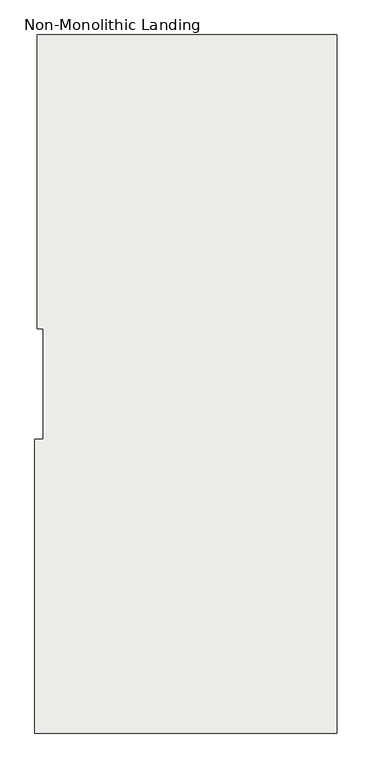
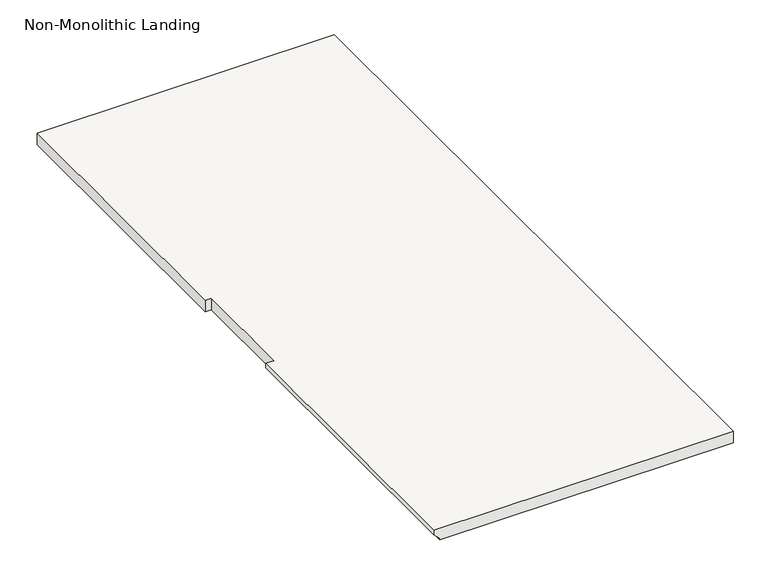
"""IFC4 building model written with IfcOpenShell, lengths in millimetres: slab geometry, Non-Monolithic Landing."""

import ifcopenshell
import ifcopenshell.guid

model = None  # the IFC model being written
_history = None  # IfcOwnerHistory: only IFC2X3 demands one
_inside = {}  # id of a spatial element -> (the spatial element, [elements in it])
_under = {}  # id of a project, library or spatial element -> (it, [spatial elements below it])
_declared = {}  # id of a project -> (the project, [libraries it declares])
_typed = {}  # id of a type object -> (the type object, [elements of that type])
_made_of = {}  # id of a material, layer set ... -> (it, [elements and type objects made of it])


def new_model(schema):
    """Start an empty IFC model of exactly this schema.

    Asked for "IFC4X3", IfcOpenShell would pick the latest addendum, in which some entities
    have other attributes; the version numbers below select the first issue.
    IFC2X3 requires an IfcOwnerHistory on every rooted entity: one is made here for all.
    """
    global model, _history
    if schema == "IFC4X3":
        model = ifcopenshell.file(schema_version=(4, 3, 0, 0))
    else:
        model = ifcopenshell.file(schema=schema)
    _inside.clear()
    _under.clear()
    _declared.clear()
    _typed.clear()
    _made_of.clear()
    _history = None
    if model.schema == "IFC2X3":
        org = make("IfcOrganization", Name="unknown")
        user = make(
            "IfcPersonAndOrganization",
            ThePerson=make("IfcPerson", FamilyName="unknown"),
            TheOrganization=org,
        )
        app = make(
            "IfcApplication",
            ApplicationDeveloper=org,
            Version="unknown",
            ApplicationFullName="unknown",
            ApplicationIdentifier="unknown",
        )
        _history = make(
            "IfcOwnerHistory",
            OwningUser=user,
            OwningApplication=app,
            ChangeAction="ADDED",
            CreationDate=0,
        )
    return model


def make(cls, **values):
    """One entity of the class cls with the attributes given. An attribute that is None is left unset."""
    return model.create_entity(
        cls, **{name: value for name, value in values.items() if value is not None}
    )


def rooted(cls, **values):
    """An entity with a GlobalId (a new one), such as an element, a storey or a relation."""
    return make(cls, GlobalId=ifcopenshell.guid.new(), OwnerHistory=_history, **values)


def si_unit(unit_type, name, prefix=None):
    """IfcSIUnit, for example si_unit("LENGTHUNIT", "METRE", prefix="MILLI")."""
    return make("IfcSIUnit", UnitType=unit_type, Prefix=prefix, Name=name)


def assignment(units):
    """IfcUnitAssignment: the units of a project."""
    return None if units is None else make("IfcUnitAssignment", Units=units)


def point(xyz):
    """IfcCartesianPoint."""
    return None if xyz is None else make("IfcCartesianPoint", Coordinates=xyz)


def direction(xyz):
    """IfcDirection."""
    return None if xyz is None else make("IfcDirection", DirectionRatios=xyz)


def frame(location, z_axis=None, x_axis=None):
    """IfcAxis2Placement3D, a coordinate frame: its origin and axes. An axis left out is left unset."""
    return make(
        "IfcAxis2Placement3D",
        Location=point(location),
        Axis=direction(z_axis),
        RefDirection=direction(x_axis),
    )


def origin():
    """The frame at (0, 0, 0) with its axes left unset."""
    return frame((0.0, 0.0, 0.0))


def place(relative_to, where):
    """IfcLocalPlacement: puts the frame where relative to a parent placement (None: the world)."""
    return make(
        "IfcLocalPlacement", PlacementRelTo=relative_to, RelativePlacement=where
    )


def context(
    kind, dimensions, precision=None, world=None, true_north=None, identifier=None
):
    """IfcGeometricRepresentationContext, for example the 3D "Model" context."""
    return make(
        "IfcGeometricRepresentationContext",
        ContextIdentifier=identifier,
        ContextType=kind,
        CoordinateSpaceDimension=dimensions,
        Precision=precision,
        WorldCoordinateSystem=world,
        TrueNorth=true_north,
    )


def project(units=None, contexts=None):
    """IfcProject with its units and contexts."""
    return rooted(
        "IfcProject",
        Name="project",
        RepresentationContexts=contexts,
        UnitsInContext=assignment(units),
    )


def spatial(cls, under=None, at=None, **own):
    """A site, building, storey or space (cls), placed at a placement, below another one or the project."""
    s = rooted(cls, ObjectPlacement=at, **own)
    if under is not None:
        _under.setdefault(under.id(), (under, []))[1].append(s)
    return s


def faces_of(points, faces, orient=None, outer=None):
    """IfcFace entities. A face is a list of loops; a loop is a list of indices into points, from 0.

    orient and outer hold one flag for each loop. By default every Orientation is true, the
    first loop of a face is its IfcFaceOuterBound and the others are IfcFaceBound.
    """
    made = []
    for i, loops in enumerate(faces):
        bounds = []
        for j, loop in enumerate(loops):
            is_outer = j == 0 if outer is None else outer[i][j]
            bounds.append(
                make(
                    "IfcFaceOuterBound" if is_outer else "IfcFaceBound",
                    Bound=make("IfcPolyLoop", Polygon=[points[k] for k in loop]),
                    Orientation=True if orient is None else orient[i][j],
                )
            )
        made.append(make("IfcFace", Bounds=bounds))
    return made


def faceted_brep(points, faces, orient=None, outer=None, voids=None):
    """IfcFacetedBrep: a solid bounded by flat faces; with voids (closed shells), ...WithVoids."""
    shared = [point(p) for p in points]
    hull = make("IfcClosedShell", CfsFaces=faces_of(shared, faces, orient, outer))
    if voids is None:
        return make("IfcFacetedBrep", Outer=hull)
    return make(
        "IfcFacetedBrepWithVoids",
        Outer=hull,
        Voids=[
            make(cls, CfsFaces=faces_of(shared, fs, o, b)) for cls, fs, o, b in voids
        ],
    )


def shape(context_of_items, identifier, shape_type, items):
    """IfcShapeRepresentation: the items that make up one representation, for example the "Body"."""
    return make(
        "IfcShapeRepresentation",
        ContextOfItems=context_of_items,
        RepresentationIdentifier=identifier,
        RepresentationType=shape_type,
        Items=items,
    )


def source(mapping_origin, context_of_items, identifier, shape_type, items):
    """IfcRepresentationMap: a shape defined once, which mapped items show again and again."""
    return make(
        "IfcRepresentationMap",
        MappingOrigin=mapping_origin,
        MappedRepresentation=shape(context_of_items, identifier, shape_type, items),
    )


def transform(
    local_origin,
    x_axis=None,
    y_axis=None,
    z_axis=None,
    scale=None,
    scale2=None,
    scale3=None,
    uniform=True,
):
    """IfcCartesianTransformationOperator3D, or its non-uniform kind. x_axis, y_axis, z_axis: its Axis1, 2, 3."""
    if uniform:
        return make(
            "IfcCartesianTransformationOperator3D",
            Axis1=direction(x_axis),
            Axis2=direction(y_axis),
            LocalOrigin=point(local_origin),
            Scale=scale,
            Axis3=direction(z_axis),
        )
    return make(
        "IfcCartesianTransformationOperator3DnonUniform",
        Axis1=direction(x_axis),
        Axis2=direction(y_axis),
        LocalOrigin=point(local_origin),
        Scale=scale,
        Axis3=direction(z_axis),
        Scale2=scale2,
        Scale3=scale3,
    )


def mapped(mapping_source, mapping_target):
    """IfcMappedItem: shows the shape of a source again, moved by a transform."""
    return make(
        "IfcMappedItem", MappingSource=mapping_source, MappingTarget=mapping_target
    )


def made_of(thing, what):
    """Note that an element or type object is made of a material, layer set ...; save() writes the relation."""
    if what is not None:
        _made_of.setdefault(what.id(), (what, []))[1].append(thing)
    return thing


def element(
    cls,
    number,
    at=None,
    inside=None,
    cuts=None,
    type_object=None,
    material=None,
    context=None,
    identifier="Body",
    shape_type=None,
    held_by="IfcProductDefinitionShape",
    body=None,
    shapes=None,
    **own,
):
    """One element of the class cls, such as IfcWall. Its Tag is "e" and its number.

    at: its placement. inside: the storey or other place that contains it. cuts: it is an
    opening in that element (IfcRelVoidsElement). A single representation is given by context,
    identifier, shape_type and body (its items); several are given by shapes. held_by: the class
    of the entity that holds the representations. save() writes the other relations.
    """
    e = rooted(cls, Tag="e%d" % number, ObjectPlacement=at, **own)
    if body is not None:
        shapes = [shape(context, identifier, shape_type, body)]
    if shapes is not None:
        e.Representation = make(held_by, Representations=shapes)
    if inside is not None:
        _inside.setdefault(inside.id(), (inside, []))[1].append(e)
    if cuts is not None:
        rooted(
            "IfcRelVoidsElement", RelatingBuildingElement=cuts, RelatedOpeningElement=e
        )
    if type_object is not None:
        _typed.setdefault(type_object.id(), (type_object, []))[1].append(e)
    return made_of(e, material)


def aggregate(whole, parts):
    """IfcRelAggregates: a whole, such as a stair, and the parts it consists of."""
    return rooted("IfcRelAggregates", RelatingObject=whole, RelatedObjects=parts)


def save(model, path):
    """Write the relations noted so far, then the file.

    IfcRelAggregates (storeys below a building ...), IfcRelContainedInSpatialStructure (elements
    in a storey), IfcRelDefinesByType, IfcRelAssociatesMaterial and IfcRelDeclares: one each for
    every whole, place, type object, material and project.
    """
    for whole, parts in _under.values():
        aggregate(whole, parts)
    for where, things in _inside.values():
        rooted(
            "IfcRelContainedInSpatialStructure",
            RelatedElements=things,
            RelatingStructure=where,
        )
    for kind, things in _typed.values():
        rooted("IfcRelDefinesByType", RelatedObjects=things, RelatingType=kind)
    for what, things in _made_of.values():
        rooted("IfcRelAssociatesMaterial", RelatedObjects=things, RelatingMaterial=what)
    for by, libraries in _declared.values():
        rooted("IfcRelDeclares", RelatingContext=by, RelatedDefinitions=libraries)
    model.write(path)


def non_monolithic_landing_eb3b7042(model_context):
    return source(origin(), model_context, "Body", "Brep", [
        faceted_brep([(20304.7956761, -8619.1304995, 32227.9065217), (20304.7956761, -8619.1304995, 32246.9565217), (20304.7956761, -7399.9304995, 32246.9565217), (20304.7956761, -7399.9304995, 32227.9065217), (20330.1956761, -8619.1304995, 32202.5065217), (20330.1956761, -7399.9304995, 32202.5065217), (21559.2045393, -8619.1304995, 32246.9565217), (21559.2045393, -5723.5304995, 32246.9565217), (20340.0045393, -5723.5304995, 32246.9565217), (20314.6045393, -5723.5304995, 32246.9565217), (20314.6045393, -6942.7304995, 32246.9565217), (20340.0045393, -6942.7304995, 32246.9565217), (20340.0045393, -7399.9304995, 32246.9565217), (20330.1956761, -8619.1304995, 32196.1565217), (20330.1956761, -7399.9304995, 32196.1565217), (20340.0045393, -7399.9304995, 32196.1565217), (20340.0045393, -6942.7304995, 32196.1565217), (20314.6045393, -6942.7304995, 32196.1565217), (20314.6045393, -5723.5304995, 32196.1565217), (20340.0045393, -5723.5304995, 32196.1565217), (21559.2045393, -5723.5304995, 32196.1565217), (21559.2045393, -8619.1304995, 32196.1565217)], [[[0, 1, 2, 3]], [[4, 0, 3, 5]], [[6, 7, 8, 9, 10, 11, 12, 2, 1]], [[13, 14, 15, 16, 17, 18, 19, 20, 21]], [[14, 13, 4, 5]], [[6, 1, 0, 4, 13, 21]], [[7, 6, 21, 20]], [[8, 7, 20, 19]], [[9, 8, 19, 18]], [[10, 9, 18, 17]], [[11, 10, 17, 16]], [[12, 11, 16, 15]], [[2, 12, 15, 14, 5, 3]]]),
    ])


if __name__ == "__main__":
    model = new_model("IFC4")
    model_context = context("Model", 3, world=origin())
    ifc_project = project(units=[si_unit("LENGTHUNIT", "METRE", prefix="MILLI")], contexts=[model_context])
    site = spatial("IfcSite", under=ifc_project)
    building = spatial("IfcBuilding", under=site)
    placement = place(None, origin())
    non_monolithic_landing_shape = non_monolithic_landing_eb3b7042(model_context)
    element("IfcSlab", 1, ObjectType="Non-Monolithic Landing", at=placement, inside=building, context=model_context, shape_type="MappedRepresentation", body=[
        mapped(non_monolithic_landing_shape, transform((0.0, 0.0, 0.0), x_axis=(1.0, 0.0, 0.0), y_axis=(0.0, 1.0, 0.0), z_axis=(0.0, 0.0, 1.0))),
    ])
    save(model, "model.ifc")
